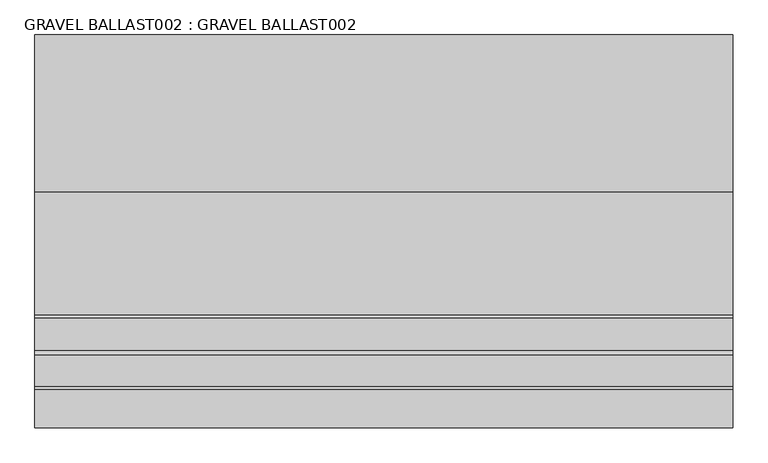
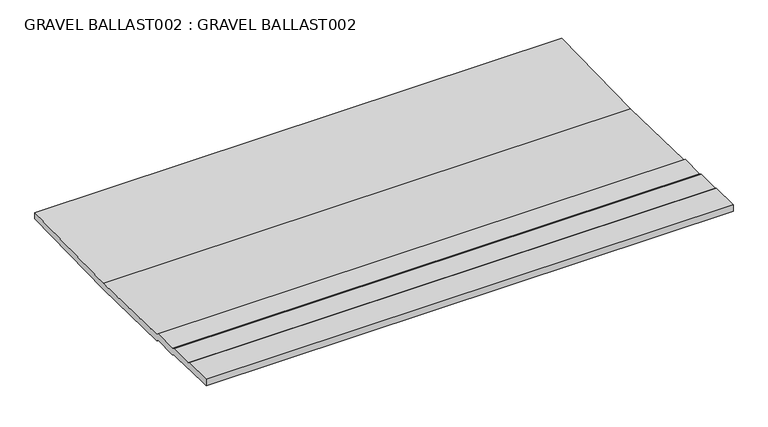
"""IFC4 building model written with IfcOpenShell, lengths in millimetres: proxy geometry, GRAVEL BALLAST002 : GRAVEL BALLAST002."""

from ifc_helpers import new_model, si_unit, frame, origin, place, context, project, spatial, polyline, outline, extrude, source, transform, mapped, element, save


def gravel_ballast002_gravel_ballast002_32d14665(model_context):
    return source(origin(), model_context, "Body", "SweptSolid", [
        extrude(outline(polyline([(-5440.365918, 40253.79375), (-5549.8654297, 40253.79375), (-5549.8654297, 40278.5320313), (-5440.365918, 40278.5320313), (-5431.6554687, 40274.2507813), (-5341.0685547, 40274.2507813), (-5328.2239153, 40268.5233193), (-5234.272168, 40270.16875), (-5225.9987305, 40262.7585938), (-4873.4420898, 40254.5398438), (-4424.6647461, 40265.496875), (-4424.6647461, 40240.7585937), (-4873.4420898, 40229.8015625), (-5225.9987305, 40238.0203125), (-5234.272168, 40245.4304687), (-5328.2239153, 40243.785038), (-5341.0685547, 40249.5125), (-5431.6554687, 40249.5125), (-5440.365918, 40253.79375)])), frame((12382.7678845, 0.0, 0.0), z_axis=(1.0, 0.0, 0.0), x_axis=(0.0, 1.0, 0.0)), (0.0, 0.0, 1.0), 2000.0),
    ])


if __name__ == "__main__":
    model = new_model("IFC4")
    model_context = context("Model", 3, world=origin())
    ifc_project = project(units=[si_unit("LENGTHUNIT", "METRE", prefix="MILLI")], contexts=[model_context])
    site = spatial("IfcSite", under=ifc_project)
    building = spatial("IfcBuilding", under=site)
    placement = place(None, origin())
    gravel_ballast002_gravel_ballast002_shape = gravel_ballast002_gravel_ballast002_32d14665(model_context)
    element("IfcBuildingElementProxy", 1, Name="GRAVEL BALLAST002 : GRAVEL BALLAST002", ObjectType="GRAVEL BALLAST002 : GRAVEL BALLAST002", at=placement, inside=building, context=model_context, shape_type="MappedRepresentation", body=[
        mapped(gravel_ballast002_gravel_ballast002_shape, transform((0.0, 0.0, 0.0), x_axis=(1.0, 0.0, 0.0), y_axis=(0.0, 1.0, 0.0), z_axis=(0.0, 0.0, 1.0))),
    ])
    save(model, "model.ifc")

# Revit data of these elements
# Type "GRAVEL BALLAST002 : GRAVEL BALLAST002"
#   NameOverride = "GRAVEL BALLAST002"
# Element 1 (IfcBuildingElementProxy, "GRAVEL BALLAST002 : GRAVEL BALLAST002")
#   Materials on its faces: "GRAVEL BALLAST"
# Materials
#   "GRAVEL BALLAST": class "Unassigned", colour RGB 128 128 128, transparency 0, Cost = 0
